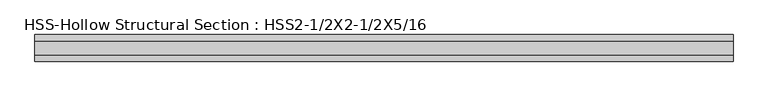
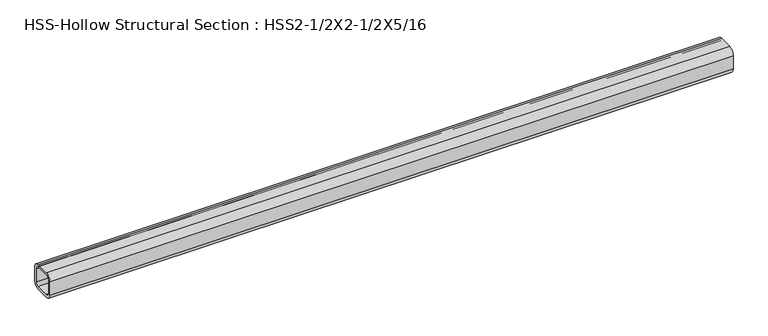
"""IFC4 building model written with IfcOpenShell, lengths in millimetres: beam geometry, HSS-Hollow Structural Section : HSS2-1/2X2-1/2X5/16."""

import ifcopenshell
import ifcopenshell.guid

model = None  # the IFC model being written
_history = None  # IfcOwnerHistory: only IFC2X3 demands one
_inside = {}  # id of a spatial element -> (the spatial element, [elements in it])
_under = {}  # id of a project, library or spatial element -> (it, [spatial elements below it])
_declared = {}  # id of a project -> (the project, [libraries it declares])
_typed = {}  # id of a type object -> (the type object, [elements of that type])
_made_of = {}  # id of a material, layer set ... -> (it, [elements and type objects made of it])


def new_model(schema):
    """Start an empty IFC model of exactly this schema.

    Asked for "IFC4X3", IfcOpenShell would pick the latest addendum, in which some entities
    have other attributes; the version numbers below select the first issue.
    IFC2X3 requires an IfcOwnerHistory on every rooted entity: one is made here for all.
    """
    global model, _history
    if schema == "IFC4X3":
        model = ifcopenshell.file(schema_version=(4, 3, 0, 0))
    else:
        model = ifcopenshell.file(schema=schema)
    _inside.clear()
    _under.clear()
    _declared.clear()
    _typed.clear()
    _made_of.clear()
    _history = None
    if model.schema == "IFC2X3":
        org = make("IfcOrganization", Name="unknown")
        user = make(
            "IfcPersonAndOrganization",
            ThePerson=make("IfcPerson", FamilyName="unknown"),
            TheOrganization=org,
        )
        app = make(
            "IfcApplication",
            ApplicationDeveloper=org,
            Version="unknown",
            ApplicationFullName="unknown",
            ApplicationIdentifier="unknown",
        )
        _history = make(
            "IfcOwnerHistory",
            OwningUser=user,
            OwningApplication=app,
            ChangeAction="ADDED",
            CreationDate=0,
        )
    return model


def make(cls, **values):
    """One entity of the class cls with the attributes given. An attribute that is None is left unset."""
    return model.create_entity(
        cls, **{name: value for name, value in values.items() if value is not None}
    )


def rooted(cls, **values):
    """An entity with a GlobalId (a new one), such as an element, a storey or a relation."""
    return make(cls, GlobalId=ifcopenshell.guid.new(), OwnerHistory=_history, **values)


def si_unit(unit_type, name, prefix=None):
    """IfcSIUnit, for example si_unit("LENGTHUNIT", "METRE", prefix="MILLI")."""
    return make("IfcSIUnit", UnitType=unit_type, Prefix=prefix, Name=name)


def assignment(units):
    """IfcUnitAssignment: the units of a project."""
    return None if units is None else make("IfcUnitAssignment", Units=units)


def point(xyz):
    """IfcCartesianPoint."""
    return None if xyz is None else make("IfcCartesianPoint", Coordinates=xyz)


def direction(xyz):
    """IfcDirection."""
    return None if xyz is None else make("IfcDirection", DirectionRatios=xyz)


def frame(location, z_axis=None, x_axis=None):
    """IfcAxis2Placement3D, a coordinate frame: its origin and axes. An axis left out is left unset."""
    return make(
        "IfcAxis2Placement3D",
        Location=point(location),
        Axis=direction(z_axis),
        RefDirection=direction(x_axis),
    )


def frame_2d(location, x_axis=None):
    """IfcAxis2Placement2D, a coordinate frame in the plane: its origin and x axis."""
    return make(
        "IfcAxis2Placement2D", Location=point(location), RefDirection=direction(x_axis)
    )


def origin():
    """The frame at (0, 0, 0) with its axes left unset."""
    return frame((0.0, 0.0, 0.0))


def place(relative_to, where):
    """IfcLocalPlacement: puts the frame where relative to a parent placement (None: the world)."""
    return make(
        "IfcLocalPlacement", PlacementRelTo=relative_to, RelativePlacement=where
    )


def context(
    kind, dimensions, precision=None, world=None, true_north=None, identifier=None
):
    """IfcGeometricRepresentationContext, for example the 3D "Model" context."""
    return make(
        "IfcGeometricRepresentationContext",
        ContextIdentifier=identifier,
        ContextType=kind,
        CoordinateSpaceDimension=dimensions,
        Precision=precision,
        WorldCoordinateSystem=world,
        TrueNorth=true_north,
    )


def project(units=None, contexts=None):
    """IfcProject with its units and contexts."""
    return rooted(
        "IfcProject",
        Name="project",
        RepresentationContexts=contexts,
        UnitsInContext=assignment(units),
    )


def spatial(cls, under=None, at=None, **own):
    """A site, building, storey or space (cls), placed at a placement, below another one or the project."""
    s = rooted(cls, ObjectPlacement=at, **own)
    if under is not None:
        _under.setdefault(under.id(), (under, []))[1].append(s)
    return s


def polyline(points):
    """IfcPolyline through the points."""
    return make("IfcPolyline", Points=[point(p) for p in points])


def circle_curve(where, radius):
    """IfcCircle in the frame where."""
    return make("IfcCircle", Position=where, Radius=radius)


def trimmed(basis, trim1, trim2, sense, master):
    """IfcTrimmedCurve: the piece of a basis curve between two trims."""
    return make(
        "IfcTrimmedCurve",
        BasisCurve=basis,
        Trim1=trim1,
        Trim2=trim2,
        SenseAgreement=sense,
        MasterRepresentation=master,
    )


def segment(curve, same_sense, transition):
    """IfcCompositeCurveSegment."""
    return make(
        "IfcCompositeCurveSegment",
        Transition=transition,
        SameSense=same_sense,
        ParentCurve=curve,
    )


def composite_curve(segments, self_intersect=None):
    """IfcCompositeCurve: segments joined end to end."""
    return make("IfcCompositeCurve", Segments=segments, SelfIntersect=self_intersect)


def outline(outer, holes=None, kind="AREA"):
    """IfcArbitraryClosedProfileDef: a profile drawn as a closed curve; with holes, ...WithVoids."""
    if holes is None:
        return make("IfcArbitraryClosedProfileDef", ProfileType=kind, OuterCurve=outer)
    return make(
        "IfcArbitraryProfileDefWithVoids",
        ProfileType=kind,
        OuterCurve=outer,
        InnerCurves=holes,
    )


def extrude(swept, where, along, depth):
    """IfcExtrudedAreaSolid: the profile swept, set in the frame where, extruded along a direction by depth."""
    return make(
        "IfcExtrudedAreaSolid",
        SweptArea=swept,
        Position=where,
        ExtrudedDirection=direction(along),
        Depth=depth,
    )


def shape(context_of_items, identifier, shape_type, items):
    """IfcShapeRepresentation: the items that make up one representation, for example the "Body"."""
    return make(
        "IfcShapeRepresentation",
        ContextOfItems=context_of_items,
        RepresentationIdentifier=identifier,
        RepresentationType=shape_type,
        Items=items,
    )


def source(mapping_origin, context_of_items, identifier, shape_type, items):
    """IfcRepresentationMap: a shape defined once, which mapped items show again and again."""
    return make(
        "IfcRepresentationMap",
        MappingOrigin=mapping_origin,
        MappedRepresentation=shape(context_of_items, identifier, shape_type, items),
    )


def transform(
    local_origin,
    x_axis=None,
    y_axis=None,
    z_axis=None,
    scale=None,
    scale2=None,
    scale3=None,
    uniform=True,
):
    """IfcCartesianTransformationOperator3D, or its non-uniform kind. x_axis, y_axis, z_axis: its Axis1, 2, 3."""
    if uniform:
        return make(
            "IfcCartesianTransformationOperator3D",
            Axis1=direction(x_axis),
            Axis2=direction(y_axis),
            LocalOrigin=point(local_origin),
            Scale=scale,
            Axis3=direction(z_axis),
        )
    return make(
        "IfcCartesianTransformationOperator3DnonUniform",
        Axis1=direction(x_axis),
        Axis2=direction(y_axis),
        LocalOrigin=point(local_origin),
        Scale=scale,
        Axis3=direction(z_axis),
        Scale2=scale2,
        Scale3=scale3,
    )


def mapped(mapping_source, mapping_target):
    """IfcMappedItem: shows the shape of a source again, moved by a transform."""
    return make(
        "IfcMappedItem", MappingSource=mapping_source, MappingTarget=mapping_target
    )


def made_of(thing, what):
    """Note that an element or type object is made of a material, layer set ...; save() writes the relation."""
    if what is not None:
        _made_of.setdefault(what.id(), (what, []))[1].append(thing)
    return thing


def element(
    cls,
    number,
    at=None,
    inside=None,
    cuts=None,
    type_object=None,
    material=None,
    context=None,
    identifier="Body",
    shape_type=None,
    held_by="IfcProductDefinitionShape",
    body=None,
    shapes=None,
    **own,
):
    """One element of the class cls, such as IfcWall. Its Tag is "e" and its number.

    at: its placement. inside: the storey or other place that contains it. cuts: it is an
    opening in that element (IfcRelVoidsElement). A single representation is given by context,
    identifier, shape_type and body (its items); several are given by shapes. held_by: the class
    of the entity that holds the representations. save() writes the other relations.
    """
    e = rooted(cls, Tag="e%d" % number, ObjectPlacement=at, **own)
    if body is not None:
        shapes = [shape(context, identifier, shape_type, body)]
    if shapes is not None:
        e.Representation = make(held_by, Representations=shapes)
    if inside is not None:
        _inside.setdefault(inside.id(), (inside, []))[1].append(e)
    if cuts is not None:
        rooted(
            "IfcRelVoidsElement", RelatingBuildingElement=cuts, RelatedOpeningElement=e
        )
    if type_object is not None:
        _typed.setdefault(type_object.id(), (type_object, []))[1].append(e)
    return made_of(e, material)


def aggregate(whole, parts):
    """IfcRelAggregates: a whole, such as a stair, and the parts it consists of."""
    return rooted("IfcRelAggregates", RelatingObject=whole, RelatedObjects=parts)


def save(model, path):
    """Write the relations noted so far, then the file.

    IfcRelAggregates (storeys below a building ...), IfcRelContainedInSpatialStructure (elements
    in a storey), IfcRelDefinesByType, IfcRelAssociatesMaterial and IfcRelDeclares: one each for
    every whole, place, type object, material and project.
    """
    for whole, parts in _under.values():
        aggregate(whole, parts)
    for where, things in _inside.values():
        rooted(
            "IfcRelContainedInSpatialStructure",
            RelatedElements=things,
            RelatingStructure=where,
        )
    for kind, things in _typed.values():
        rooted("IfcRelDefinesByType", RelatedObjects=things, RelatingType=kind)
    for what, things in _made_of.values():
        rooted("IfcRelAssociatesMaterial", RelatedObjects=things, RelatingMaterial=what)
    for by, libraries in _declared.values():
        rooted("IfcRelDeclares", RelatingContext=by, RelatedDefinitions=libraries)
    model.write(path)


def hss_hollow_structural_section_hss2_1_2x2_1_2x5_16_c579bad2(model_context):
    return source(origin(), model_context, "Body", "SweptSolid", [
        extrude(outline(composite_curve([segment(polyline([(31.75, 16.9672), (31.75, -16.9672)]), True, "CONTINUOUS"), segment(trimmed(circle_curve(frame_2d((16.9672, -16.9672)), 14.7828), [point((31.75, -16.9672))], [point((16.9672, -31.75))], False, "CARTESIAN"), True, "CONTINUOUS"), segment(polyline([(16.9672, -31.75), (-16.9672, -31.75)]), True, "CONTINUOUS"), segment(trimmed(circle_curve(frame_2d((-16.9672, -16.9672)), 14.7828), [point((-16.9672, -31.75))], [point((-31.75, -16.9672))], False, "CARTESIAN"), True, "CONTINUOUS"), segment(polyline([(-31.75, -16.9672), (-31.75, 16.9672)]), True, "CONTINUOUS"), segment(trimmed(circle_curve(frame_2d((-16.9672, 16.9672)), 14.7828), [point((-31.75, 16.9672))], [point((-16.9672, 31.75))], False, "CARTESIAN"), True, "CONTINUOUS"), segment(polyline([(-16.9672, 31.75), (16.9672, 31.75)]), True, "CONTINUOUS"), segment(trimmed(circle_curve(frame_2d((16.9672, 16.9672)), 14.7828), [point((16.9672, 31.75))], [point((31.75, 16.9672))], False, "CARTESIAN"), True, "CONTINUOUS")], self_intersect=False), holes=[composite_curve([segment(trimmed(circle_curve(frame_2d((-16.9672, 16.9672)), 7.3914), [point((-16.9672, 24.3586))], [point((-24.3586, 16.9672))], True, "CARTESIAN"), True, "CONTINUOUS"), segment(polyline([(-24.3586, 16.9672), (-24.3586, -16.9672)]), True, "CONTINUOUS"), segment(trimmed(circle_curve(frame_2d((-16.9672, -16.9672)), 7.3914), [point((-24.3586, -16.9672))], [point((-16.9672, -24.3586))], True, "CARTESIAN"), True, "CONTINUOUS"), segment(polyline([(-16.9672, -24.3586), (16.9672, -24.3586)]), True, "CONTINUOUS"), segment(trimmed(circle_curve(frame_2d((16.9672, -16.9672)), 7.3914), [point((16.9672, -24.3586))], [point((24.3586, -16.9672))], True, "CARTESIAN"), True, "CONTINUOUS"), segment(polyline([(24.3586, -16.9672), (24.3586, 16.9672)]), True, "CONTINUOUS"), segment(trimmed(circle_curve(frame_2d((16.9672, 16.9672)), 7.3914), [point((24.3586, 16.9672))], [point((16.9672, 24.3586))], True, "CARTESIAN"), True, "CONTINUOUS"), segment(polyline([(16.9672, 24.3586), (-16.9672, 24.3586)]), True, "CONTINUOUS")], self_intersect=False)]), frame((-812.927, 0.0, 0.0), z_axis=(1.0, 0.0, 0.0), x_axis=(0.0, 1.0, 0.0)), (0.0, 0.0, 1.0), 1663.7),
    ])


if __name__ == "__main__":
    model = new_model("IFC4")
    model_context = context("Model", 3, world=origin())
    ifc_project = project(units=[si_unit("LENGTHUNIT", "METRE", prefix="MILLI")], contexts=[model_context])
    site = spatial("IfcSite", under=ifc_project)
    building = spatial("IfcBuilding", under=site)
    placement = place(None, origin())
    hss_hollow_structural_section_hss2_1_2x2_1_2x5_16_shape = hss_hollow_structural_section_hss2_1_2x2_1_2x5_16_c579bad2(model_context)
    element("IfcBeam", 1, ObjectType="HSS-Hollow Structural Section : HSS2-1/2X2-1/2X5/16", at=placement, inside=building, context=model_context, shape_type="MappedRepresentation", body=[
        mapped(hss_hollow_structural_section_hss2_1_2x2_1_2x5_16_shape, transform((0.0, 0.0, 0.0), x_axis=(1.0, 0.0, 0.0), y_axis=(0.0, 1.0, 0.0), z_axis=(0.0, 0.0, 1.0))),
    ])
    save(model, "model.ifc")

# Revit data of these elements
# Type "HSS-Hollow Structural Section : HSS2-1/2X2-1/2X5/16"
#   Assembly Code = "B10"
#   Shape = "Square"
#   W = 8.4
#   Ht = 0' - 2 1/2"
#   Length [instance default] = 5' - 0"
#   b = 0' - 2 1/2"
#   kr = 0' - 0.582"
#   t = 0' - 0.291"
#   A = 0.0163194 SF
#   Structural Material [instance default] = Steel ASTM A500, Grade B, Rectangular and Square
# Element 1 (IfcBeam, "HSS-Hollow Structural Section : HSS2-1/2X2-1/2X5/16")
#   Materials on its faces: "Steel ASTM A500, Grade B, Rectangular and Square"
# Materials
#   "Steel ASTM A500, Grade B, Rectangular and Square": class "Metal", colour RGB 199 199 199, transparency 0, Description = "Carbon steel", Cost = 0
